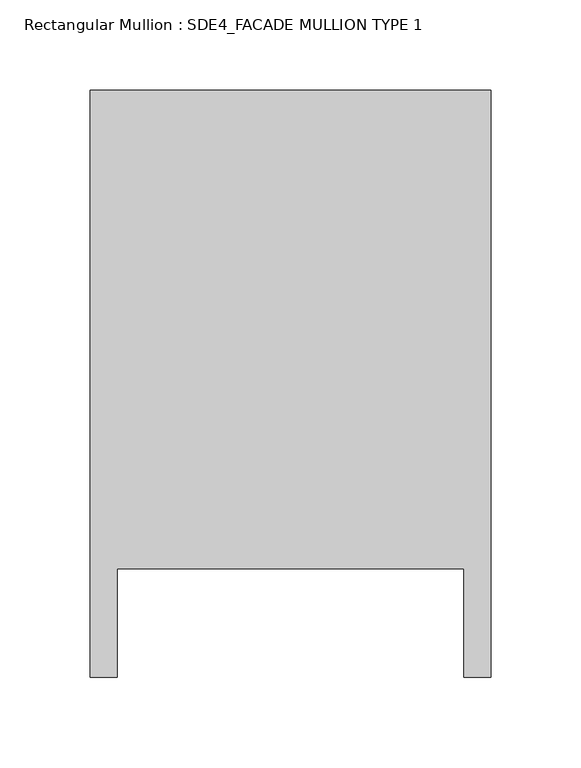
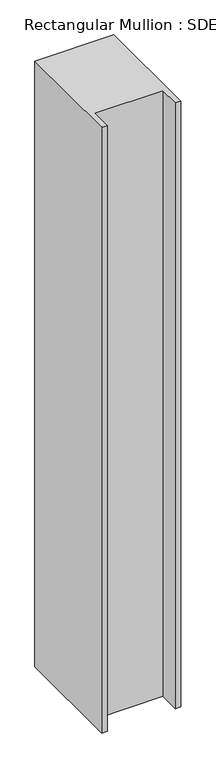
"""IFC4 building model written with IfcOpenShell, lengths in millimetres: member geometry, Rectangular Mullion : SDE4_FACADE MULLION TYPE 1."""

from ifc_helpers import new_model, si_unit, frame, origin, place, context, project, spatial, polyline, outline, extrude, source, transform, mapped, element, save


def rectangular_mullion_sde4_facade_mullion_type_1_8e626999(model_context):
    return source(origin(), model_context, "Body", "SweptSolid", [
        extrude(outline(polyline([(111.0, 132.5), (111.0, -192.5), (96.0, -192.5), (96.0, -132.5), (-96.0, -132.5), (-96.0, -192.5), (-111.0, -192.5), (-111.0, 132.5), (111.0, 132.5)])), frame((0.0, 0.0, -1800.0), z_axis=(0.0, 0.0, 1.0), x_axis=(1.0, 0.0, 0.0)), (0.0, 0.0, 1.0), 1800.0),
    ])


if __name__ == "__main__":
    model = new_model("IFC4")
    model_context = context("Model", 3, world=origin())
    ifc_project = project(units=[si_unit("LENGTHUNIT", "METRE", prefix="MILLI")], contexts=[model_context])
    site = spatial("IfcSite", under=ifc_project)
    building = spatial("IfcBuilding", under=site)
    placement = place(None, origin())
    rectangular_mullion_sde4_facade_mullion_type_1_shape = rectangular_mullion_sde4_facade_mullion_type_1_8e626999(model_context)
    element("IfcMember", 1, ObjectType="Rectangular Mullion : SDE4_FACADE MULLION TYPE 1", at=placement, inside=building, context=model_context, shape_type="MappedRepresentation", body=[
        mapped(rectangular_mullion_sde4_facade_mullion_type_1_shape, transform((0.0, 0.0, 0.0), x_axis=(1.0, 0.0, 0.0), y_axis=(0.0, 1.0, 0.0), z_axis=(0.0, 0.0, 1.0))),
    ])
    save(model, "model.ifc")

# Revit data of these elements
# Type "Rectangular Mullion : SDE4_FACADE MULLION TYPE 1"
#   built-in parameter 1007322 = 0.869423 (stored number, unit not read)
#   built-in parameter 1007321 = 0.364173 (stored number, unit not read)
#   built-in parameter 1007320 = 0.364173 (stored number, unit not read)
